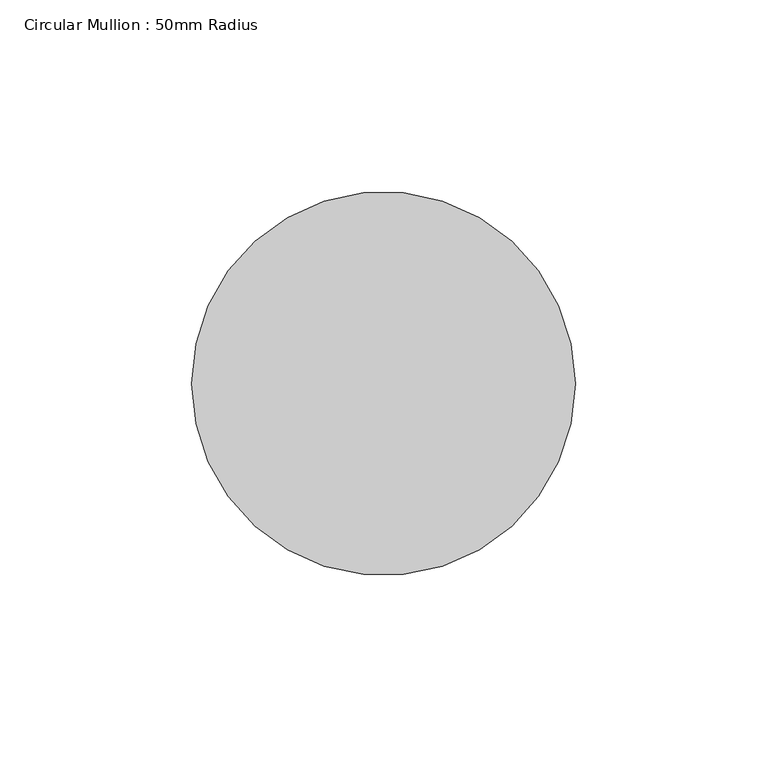
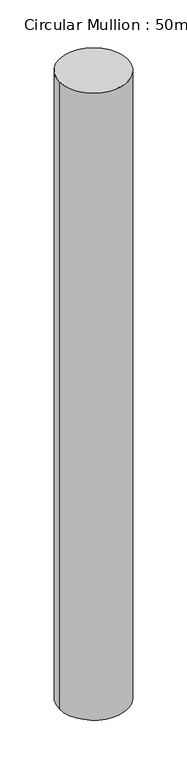
"""IFC4 building model written with IfcOpenShell, lengths in millimetres: member geometry, Circular Mullion : 50mm Radius."""

import ifcopenshell
import ifcopenshell.guid

model = None  # the IFC model being written
_history = None  # IfcOwnerHistory: only IFC2X3 demands one
_inside = {}  # id of a spatial element -> (the spatial element, [elements in it])
_under = {}  # id of a project, library or spatial element -> (it, [spatial elements below it])
_declared = {}  # id of a project -> (the project, [libraries it declares])
_typed = {}  # id of a type object -> (the type object, [elements of that type])
_made_of = {}  # id of a material, layer set ... -> (it, [elements and type objects made of it])


def new_model(schema):
    """Start an empty IFC model of exactly this schema.

    Asked for "IFC4X3", IfcOpenShell would pick the latest addendum, in which some entities
    have other attributes; the version numbers below select the first issue.
    IFC2X3 requires an IfcOwnerHistory on every rooted entity: one is made here for all.
    """
    global model, _history
    if schema == "IFC4X3":
        model = ifcopenshell.file(schema_version=(4, 3, 0, 0))
    else:
        model = ifcopenshell.file(schema=schema)
    _inside.clear()
    _under.clear()
    _declared.clear()
    _typed.clear()
    _made_of.clear()
    _history = None
    if model.schema == "IFC2X3":
        org = make("IfcOrganization", Name="unknown")
        user = make(
            "IfcPersonAndOrganization",
            ThePerson=make("IfcPerson", FamilyName="unknown"),
            TheOrganization=org,
        )
        app = make(
            "IfcApplication",
            ApplicationDeveloper=org,
            Version="unknown",
            ApplicationFullName="unknown",
            ApplicationIdentifier="unknown",
        )
        _history = make(
            "IfcOwnerHistory",
            OwningUser=user,
            OwningApplication=app,
            ChangeAction="ADDED",
            CreationDate=0,
        )
    return model


def make(cls, **values):
    """One entity of the class cls with the attributes given. An attribute that is None is left unset."""
    return model.create_entity(
        cls, **{name: value for name, value in values.items() if value is not None}
    )


def rooted(cls, **values):
    """An entity with a GlobalId (a new one), such as an element, a storey or a relation."""
    return make(cls, GlobalId=ifcopenshell.guid.new(), OwnerHistory=_history, **values)


def si_unit(unit_type, name, prefix=None):
    """IfcSIUnit, for example si_unit("LENGTHUNIT", "METRE", prefix="MILLI")."""
    return make("IfcSIUnit", UnitType=unit_type, Prefix=prefix, Name=name)


def assignment(units):
    """IfcUnitAssignment: the units of a project."""
    return None if units is None else make("IfcUnitAssignment", Units=units)


def point(xyz):
    """IfcCartesianPoint."""
    return None if xyz is None else make("IfcCartesianPoint", Coordinates=xyz)


def direction(xyz):
    """IfcDirection."""
    return None if xyz is None else make("IfcDirection", DirectionRatios=xyz)


def frame(location, z_axis=None, x_axis=None):
    """IfcAxis2Placement3D, a coordinate frame: its origin and axes. An axis left out is left unset."""
    return make(
        "IfcAxis2Placement3D",
        Location=point(location),
        Axis=direction(z_axis),
        RefDirection=direction(x_axis),
    )


def frame_2d(location, x_axis=None):
    """IfcAxis2Placement2D, a coordinate frame in the plane: its origin and x axis."""
    return make(
        "IfcAxis2Placement2D", Location=point(location), RefDirection=direction(x_axis)
    )


def origin():
    """The frame at (0, 0, 0) with its axes left unset."""
    return frame((0.0, 0.0, 0.0))


def origin_2d():
    """The frame at (0, 0) in the plane with its x axis left unset."""
    return frame_2d((0.0, 0.0))


def place(relative_to, where):
    """IfcLocalPlacement: puts the frame where relative to a parent placement (None: the world)."""
    return make(
        "IfcLocalPlacement", PlacementRelTo=relative_to, RelativePlacement=where
    )


def context(
    kind, dimensions, precision=None, world=None, true_north=None, identifier=None
):
    """IfcGeometricRepresentationContext, for example the 3D "Model" context."""
    return make(
        "IfcGeometricRepresentationContext",
        ContextIdentifier=identifier,
        ContextType=kind,
        CoordinateSpaceDimension=dimensions,
        Precision=precision,
        WorldCoordinateSystem=world,
        TrueNorth=true_north,
    )


def project(units=None, contexts=None):
    """IfcProject with its units and contexts."""
    return rooted(
        "IfcProject",
        Name="project",
        RepresentationContexts=contexts,
        UnitsInContext=assignment(units),
    )


def spatial(cls, under=None, at=None, **own):
    """A site, building, storey or space (cls), placed at a placement, below another one or the project."""
    s = rooted(cls, ObjectPlacement=at, **own)
    if under is not None:
        _under.setdefault(under.id(), (under, []))[1].append(s)
    return s


def circle_curve(where, radius):
    """IfcCircle in the frame where."""
    return make("IfcCircle", Position=where, Radius=radius)


def trimmed(basis, trim1, trim2, sense, master):
    """IfcTrimmedCurve: the piece of a basis curve between two trims."""
    return make(
        "IfcTrimmedCurve",
        BasisCurve=basis,
        Trim1=trim1,
        Trim2=trim2,
        SenseAgreement=sense,
        MasterRepresentation=master,
    )


def segment(curve, same_sense, transition):
    """IfcCompositeCurveSegment."""
    return make(
        "IfcCompositeCurveSegment",
        Transition=transition,
        SameSense=same_sense,
        ParentCurve=curve,
    )


def composite_curve(segments, self_intersect=None):
    """IfcCompositeCurve: segments joined end to end."""
    return make("IfcCompositeCurve", Segments=segments, SelfIntersect=self_intersect)


def outline(outer, holes=None, kind="AREA"):
    """IfcArbitraryClosedProfileDef: a profile drawn as a closed curve; with holes, ...WithVoids."""
    if holes is None:
        return make("IfcArbitraryClosedProfileDef", ProfileType=kind, OuterCurve=outer)
    return make(
        "IfcArbitraryProfileDefWithVoids",
        ProfileType=kind,
        OuterCurve=outer,
        InnerCurves=holes,
    )


def extrude(swept, where, along, depth):
    """IfcExtrudedAreaSolid: the profile swept, set in the frame where, extruded along a direction by depth."""
    return make(
        "IfcExtrudedAreaSolid",
        SweptArea=swept,
        Position=where,
        ExtrudedDirection=direction(along),
        Depth=depth,
    )


def shape(context_of_items, identifier, shape_type, items):
    """IfcShapeRepresentation: the items that make up one representation, for example the "Body"."""
    return make(
        "IfcShapeRepresentation",
        ContextOfItems=context_of_items,
        RepresentationIdentifier=identifier,
        RepresentationType=shape_type,
        Items=items,
    )


def source(mapping_origin, context_of_items, identifier, shape_type, items):
    """IfcRepresentationMap: a shape defined once, which mapped items show again and again."""
    return make(
        "IfcRepresentationMap",
        MappingOrigin=mapping_origin,
        MappedRepresentation=shape(context_of_items, identifier, shape_type, items),
    )


def transform(
    local_origin,
    x_axis=None,
    y_axis=None,
    z_axis=None,
    scale=None,
    scale2=None,
    scale3=None,
    uniform=True,
):
    """IfcCartesianTransformationOperator3D, or its non-uniform kind. x_axis, y_axis, z_axis: its Axis1, 2, 3."""
    if uniform:
        return make(
            "IfcCartesianTransformationOperator3D",
            Axis1=direction(x_axis),
            Axis2=direction(y_axis),
            LocalOrigin=point(local_origin),
            Scale=scale,
            Axis3=direction(z_axis),
        )
    return make(
        "IfcCartesianTransformationOperator3DnonUniform",
        Axis1=direction(x_axis),
        Axis2=direction(y_axis),
        LocalOrigin=point(local_origin),
        Scale=scale,
        Axis3=direction(z_axis),
        Scale2=scale2,
        Scale3=scale3,
    )


def mapped(mapping_source, mapping_target):
    """IfcMappedItem: shows the shape of a source again, moved by a transform."""
    return make(
        "IfcMappedItem", MappingSource=mapping_source, MappingTarget=mapping_target
    )


def made_of(thing, what):
    """Note that an element or type object is made of a material, layer set ...; save() writes the relation."""
    if what is not None:
        _made_of.setdefault(what.id(), (what, []))[1].append(thing)
    return thing


def element(
    cls,
    number,
    at=None,
    inside=None,
    cuts=None,
    type_object=None,
    material=None,
    context=None,
    identifier="Body",
    shape_type=None,
    held_by="IfcProductDefinitionShape",
    body=None,
    shapes=None,
    **own,
):
    """One element of the class cls, such as IfcWall. Its Tag is "e" and its number.

    at: its placement. inside: the storey or other place that contains it. cuts: it is an
    opening in that element (IfcRelVoidsElement). A single representation is given by context,
    identifier, shape_type and body (its items); several are given by shapes. held_by: the class
    of the entity that holds the representations. save() writes the other relations.
    """
    e = rooted(cls, Tag="e%d" % number, ObjectPlacement=at, **own)
    if body is not None:
        shapes = [shape(context, identifier, shape_type, body)]
    if shapes is not None:
        e.Representation = make(held_by, Representations=shapes)
    if inside is not None:
        _inside.setdefault(inside.id(), (inside, []))[1].append(e)
    if cuts is not None:
        rooted(
            "IfcRelVoidsElement", RelatingBuildingElement=cuts, RelatedOpeningElement=e
        )
    if type_object is not None:
        _typed.setdefault(type_object.id(), (type_object, []))[1].append(e)
    return made_of(e, material)


def aggregate(whole, parts):
    """IfcRelAggregates: a whole, such as a stair, and the parts it consists of."""
    return rooted("IfcRelAggregates", RelatingObject=whole, RelatedObjects=parts)


def save(model, path):
    """Write the relations noted so far, then the file.

    IfcRelAggregates (storeys below a building ...), IfcRelContainedInSpatialStructure (elements
    in a storey), IfcRelDefinesByType, IfcRelAssociatesMaterial and IfcRelDeclares: one each for
    every whole, place, type object, material and project.
    """
    for whole, parts in _under.values():
        aggregate(whole, parts)
    for where, things in _inside.values():
        rooted(
            "IfcRelContainedInSpatialStructure",
            RelatedElements=things,
            RelatingStructure=where,
        )
    for kind, things in _typed.values():
        rooted("IfcRelDefinesByType", RelatedObjects=things, RelatingType=kind)
    for what, things in _made_of.values():
        rooted("IfcRelAssociatesMaterial", RelatedObjects=things, RelatingMaterial=what)
    for by, libraries in _declared.values():
        rooted("IfcRelDeclares", RelatingContext=by, RelatedDefinitions=libraries)
    model.write(path)


def circular_mullion_50mm_radius_2d9f92fa(model_context):
    return source(origin(), model_context, "Body", "SweptSolid", [
        extrude(outline(composite_curve([segment(trimmed(circle_curve(origin_2d(), 50.0), [point((50.0, 0.0))], [point((-50.0, 0.0))], False, "CARTESIAN"), True, "CONTINUOUS"), segment(trimmed(circle_curve(origin_2d(), 50.0), [point((-50.0, 0.0))], [point((50.0, 0.0))], False, "CARTESIAN"), True, "CONTINUOUS")], self_intersect=False)), frame((0.0, 0.0, -969.2993351), z_axis=(0.0, 0.0, 1.0), x_axis=(1.0, 0.0, 0.0)), (0.0, 0.0, 1.0), 969.2993351),
    ])


if __name__ == "__main__":
    model = new_model("IFC4")
    model_context = context("Model", 3, world=origin())
    ifc_project = project(units=[si_unit("LENGTHUNIT", "METRE", prefix="MILLI")], contexts=[model_context])
    site = spatial("IfcSite", under=ifc_project)
    building = spatial("IfcBuilding", under=site)
    placement = place(None, origin())
    circular_mullion_50mm_radius_shape = circular_mullion_50mm_radius_2d9f92fa(model_context)
    element("IfcMember", 1, ObjectType="Circular Mullion : 50mm Radius", at=placement, inside=building, context=model_context, shape_type="MappedRepresentation", body=[
        mapped(circular_mullion_50mm_radius_shape, transform((0.0, 0.0, 0.0), x_axis=(1.0, 0.0, 0.0), y_axis=(0.0, 1.0, 0.0), z_axis=(0.0, 0.0, 1.0))),
    ])
    save(model, "model.ifc")

# Revit data of these elements
# Type "Circular Mullion : 50mm Radius"
#   built-in parameter 1007350 = 0.164042 (stored number, unit not read)
# Element 1 (IfcMember, "Circular Mullion : 50mm Radius")
#   Materials on its faces: "Aluminium"
# Materials
#   "Aluminium": class "Metal", colour RGB 247 247 247, transparency 0, Description = "Aluminium 6061", Cost = 0
